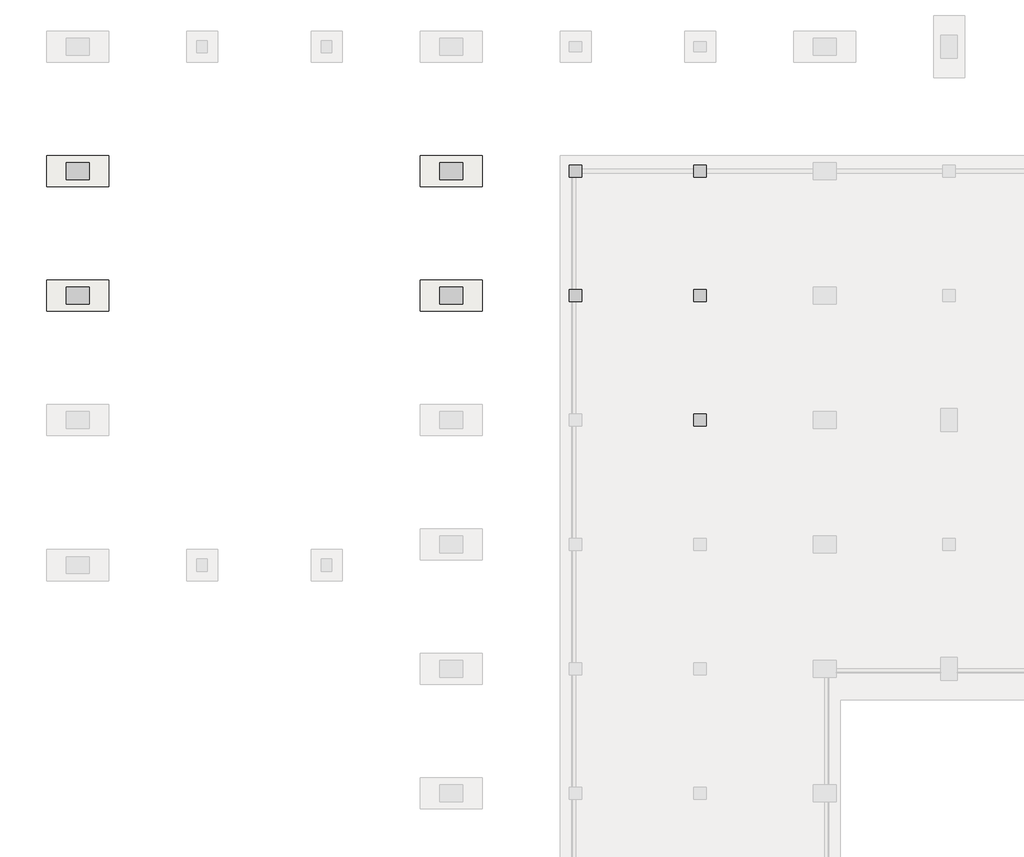
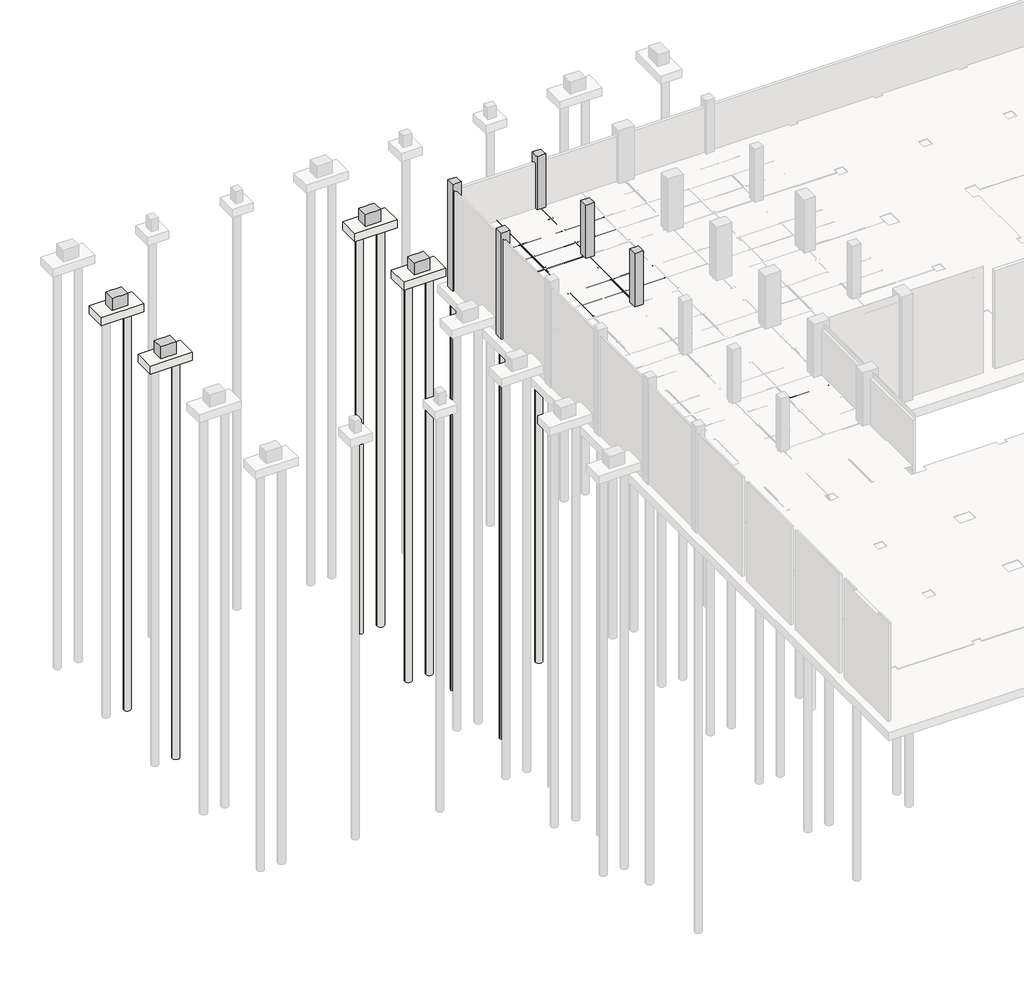
# Not in any storey, part 8 of 16: 24 beams, 13 slabs, 9 columns.
"""IFC4 building model written with IfcOpenShell, lengths in millimetres."""

import ifcopenshell
import ifcopenshell.guid

model = None  # the IFC model being written
_history = None  # IfcOwnerHistory: only IFC2X3 demands one
_inside = {}  # id of a spatial element -> (the spatial element, [elements in it])
_under = {}  # id of a project, library or spatial element -> (it, [spatial elements below it])
_declared = {}  # id of a project -> (the project, [libraries it declares])
_typed = {}  # id of a type object -> (the type object, [elements of that type])
_made_of = {}  # id of a material, layer set ... -> (it, [elements and type objects made of it])


def new_model(schema):
    """Start an empty IFC model of exactly this schema.

    Asked for "IFC4X3", IfcOpenShell would pick the latest addendum, in which some entities
    have other attributes; the version numbers below select the first issue.
    IFC2X3 requires an IfcOwnerHistory on every rooted entity: one is made here for all.
    """
    global model, _history
    if schema == "IFC4X3":
        model = ifcopenshell.file(schema_version=(4, 3, 0, 0))
    else:
        model = ifcopenshell.file(schema=schema)
    _inside.clear()
    _under.clear()
    _declared.clear()
    _typed.clear()
    _made_of.clear()
    _history = None
    if model.schema == "IFC2X3":
        org = make("IfcOrganization", Name="unknown")
        user = make(
            "IfcPersonAndOrganization",
            ThePerson=make("IfcPerson", FamilyName="unknown"),
            TheOrganization=org,
        )
        app = make(
            "IfcApplication",
            ApplicationDeveloper=org,
            Version="unknown",
            ApplicationFullName="unknown",
            ApplicationIdentifier="unknown",
        )
        _history = make(
            "IfcOwnerHistory",
            OwningUser=user,
            OwningApplication=app,
            ChangeAction="ADDED",
            CreationDate=0,
        )
    return model


def make(cls, **values):
    """One entity of the class cls with the attributes given. An attribute that is None is left unset."""
    return model.create_entity(
        cls, **{name: value for name, value in values.items() if value is not None}
    )


def rooted(cls, **values):
    """An entity with a GlobalId (a new one), such as an element, a storey or a relation."""
    return make(cls, GlobalId=ifcopenshell.guid.new(), OwnerHistory=_history, **values)


def si_unit(unit_type, name, prefix=None):
    """IfcSIUnit, for example si_unit("LENGTHUNIT", "METRE", prefix="MILLI")."""
    return make("IfcSIUnit", UnitType=unit_type, Prefix=prefix, Name=name)


def assignment(units):
    """IfcUnitAssignment: the units of a project."""
    return None if units is None else make("IfcUnitAssignment", Units=units)


def point(xyz):
    """IfcCartesianPoint."""
    return None if xyz is None else make("IfcCartesianPoint", Coordinates=xyz)


def direction(xyz):
    """IfcDirection."""
    return None if xyz is None else make("IfcDirection", DirectionRatios=xyz)


def frame(location, z_axis=None, x_axis=None):
    """IfcAxis2Placement3D, a coordinate frame: its origin and axes. An axis left out is left unset."""
    return make(
        "IfcAxis2Placement3D",
        Location=point(location),
        Axis=direction(z_axis),
        RefDirection=direction(x_axis),
    )


def frame_2d(location, x_axis=None):
    """IfcAxis2Placement2D, a coordinate frame in the plane: its origin and x axis."""
    return make(
        "IfcAxis2Placement2D", Location=point(location), RefDirection=direction(x_axis)
    )


def origin():
    """The frame at (0, 0, 0) with its axes left unset."""
    return frame((0.0, 0.0, 0.0))


def place(relative_to, where):
    """IfcLocalPlacement: puts the frame where relative to a parent placement (None: the world)."""
    return make(
        "IfcLocalPlacement", PlacementRelTo=relative_to, RelativePlacement=where
    )


def context(
    kind, dimensions, precision=None, world=None, true_north=None, identifier=None
):
    """IfcGeometricRepresentationContext, for example the 3D "Model" context."""
    return make(
        "IfcGeometricRepresentationContext",
        ContextIdentifier=identifier,
        ContextType=kind,
        CoordinateSpaceDimension=dimensions,
        Precision=precision,
        WorldCoordinateSystem=world,
        TrueNorth=true_north,
    )


def project(units=None, contexts=None):
    """IfcProject with its units and contexts."""
    return rooted(
        "IfcProject",
        Name="project",
        RepresentationContexts=contexts,
        UnitsInContext=assignment(units),
    )


def spatial(cls, under=None, at=None, **own):
    """A site, building, storey or space (cls), placed at a placement, below another one or the project."""
    s = rooted(cls, ObjectPlacement=at, **own)
    if under is not None:
        _under.setdefault(under.id(), (under, []))[1].append(s)
    return s


def polyline(points):
    """IfcPolyline through the points."""
    return make("IfcPolyline", Points=[point(p) for p in points])


def circle_curve(where, radius):
    """IfcCircle in the frame where."""
    return make("IfcCircle", Position=where, Radius=radius)


def trimmed(basis, trim1, trim2, sense, master):
    """IfcTrimmedCurve: the piece of a basis curve between two trims."""
    return make(
        "IfcTrimmedCurve",
        BasisCurve=basis,
        Trim1=trim1,
        Trim2=trim2,
        SenseAgreement=sense,
        MasterRepresentation=master,
    )


def segment(curve, same_sense, transition):
    """IfcCompositeCurveSegment."""
    return make(
        "IfcCompositeCurveSegment",
        Transition=transition,
        SameSense=same_sense,
        ParentCurve=curve,
    )


def composite_curve(segments, self_intersect=None):
    """IfcCompositeCurve: segments joined end to end."""
    return make("IfcCompositeCurve", Segments=segments, SelfIntersect=self_intersect)


def outline(outer, holes=None, kind="AREA"):
    """IfcArbitraryClosedProfileDef: a profile drawn as a closed curve; with holes, ...WithVoids."""
    if holes is None:
        return make("IfcArbitraryClosedProfileDef", ProfileType=kind, OuterCurve=outer)
    return make(
        "IfcArbitraryProfileDefWithVoids",
        ProfileType=kind,
        OuterCurve=outer,
        InnerCurves=holes,
    )


def extrude(swept, where, along, depth):
    """IfcExtrudedAreaSolid: the profile swept, set in the frame where, extruded along a direction by depth."""
    return make(
        "IfcExtrudedAreaSolid",
        SweptArea=swept,
        Position=where,
        ExtrudedDirection=direction(along),
        Depth=depth,
    )


def faces_of(points, faces, orient=None, outer=None):
    """IfcFace entities. A face is a list of loops; a loop is a list of indices into points, from 0.

    orient and outer hold one flag for each loop. By default every Orientation is true, the
    first loop of a face is its IfcFaceOuterBound and the others are IfcFaceBound.
    """
    made = []
    for i, loops in enumerate(faces):
        bounds = []
        for j, loop in enumerate(loops):
            is_outer = j == 0 if outer is None else outer[i][j]
            bounds.append(
                make(
                    "IfcFaceOuterBound" if is_outer else "IfcFaceBound",
                    Bound=make("IfcPolyLoop", Polygon=[points[k] for k in loop]),
                    Orientation=True if orient is None else orient[i][j],
                )
            )
        made.append(make("IfcFace", Bounds=bounds))
    return made


def faceted_brep(points, faces, orient=None, outer=None, voids=None):
    """IfcFacetedBrep: a solid bounded by flat faces; with voids (closed shells), ...WithVoids."""
    shared = [point(p) for p in points]
    hull = make("IfcClosedShell", CfsFaces=faces_of(shared, faces, orient, outer))
    if voids is None:
        return make("IfcFacetedBrep", Outer=hull)
    return make(
        "IfcFacetedBrepWithVoids",
        Outer=hull,
        Voids=[
            make(cls, CfsFaces=faces_of(shared, fs, o, b)) for cls, fs, o, b in voids
        ],
    )


def shape(context_of_items, identifier, shape_type, items):
    """IfcShapeRepresentation: the items that make up one representation, for example the "Body"."""
    return make(
        "IfcShapeRepresentation",
        ContextOfItems=context_of_items,
        RepresentationIdentifier=identifier,
        RepresentationType=shape_type,
        Items=items,
    )


def made_of(thing, what):
    """Note that an element or type object is made of a material, layer set ...; save() writes the relation."""
    if what is not None:
        _made_of.setdefault(what.id(), (what, []))[1].append(thing)
    return thing


def element(
    cls,
    number,
    at=None,
    inside=None,
    cuts=None,
    type_object=None,
    material=None,
    context=None,
    identifier="Body",
    shape_type=None,
    held_by="IfcProductDefinitionShape",
    body=None,
    shapes=None,
    **own,
):
    """One element of the class cls, such as IfcWall. Its Tag is "e" and its number.

    at: its placement. inside: the storey or other place that contains it. cuts: it is an
    opening in that element (IfcRelVoidsElement). A single representation is given by context,
    identifier, shape_type and body (its items); several are given by shapes. held_by: the class
    of the entity that holds the representations. save() writes the other relations.
    """
    e = rooted(cls, Tag="e%d" % number, ObjectPlacement=at, **own)
    if body is not None:
        shapes = [shape(context, identifier, shape_type, body)]
    if shapes is not None:
        e.Representation = make(held_by, Representations=shapes)
    if inside is not None:
        _inside.setdefault(inside.id(), (inside, []))[1].append(e)
    if cuts is not None:
        rooted(
            "IfcRelVoidsElement", RelatingBuildingElement=cuts, RelatedOpeningElement=e
        )
    if type_object is not None:
        _typed.setdefault(type_object.id(), (type_object, []))[1].append(e)
    return made_of(e, material)


def aggregate(whole, parts):
    """IfcRelAggregates: a whole, such as a stair, and the parts it consists of."""
    return rooted("IfcRelAggregates", RelatingObject=whole, RelatedObjects=parts)


def save(model, path):
    """Write the relations noted so far, then the file.

    IfcRelAggregates (storeys below a building ...), IfcRelContainedInSpatialStructure (elements
    in a storey), IfcRelDefinesByType, IfcRelAssociatesMaterial and IfcRelDeclares: one each for
    every whole, place, type object, material and project.
    """
    for whole, parts in _under.values():
        aggregate(whole, parts)
    for where, things in _inside.values():
        rooted(
            "IfcRelContainedInSpatialStructure",
            RelatedElements=things,
            RelatingStructure=where,
        )
    for kind, things in _typed.values():
        rooted("IfcRelDefinesByType", RelatedObjects=things, RelatingType=kind)
    for what, things in _made_of.values():
        rooted("IfcRelAssociatesMaterial", RelatedObjects=things, RelatingMaterial=what)
    for by, libraries in _declared.values():
        rooted("IfcRelDeclares", RelatingContext=by, RelatedDefinitions=libraries)
    model.write(path)


model = new_model("IFC4")

# Units and contexts
model_context = context("Model", 3, world=origin())
ifc_project = project(units=[si_unit("LENGTHUNIT", "METRE", prefix="MILLI")], contexts=[model_context])

# Site, building
site = spatial("IfcSite", under=ifc_project)
building = spatial("IfcBuilding", under=site)

# Beams
placement = place(None, origin())
element("IfcBeam", 1, at=placement, inside=building, context=model_context, shape_type="SweptSolid", body=[
    extrude(outline(composite_curve([segment(polyline([(-11900.0, -4187.0381366), (-11900.0, -4200.0381366), (-12100.0, -4200.0381366), (-12100.0, -4187.0381366), (-12020.0, -4187.0381366)]), True, "CONTINUOUS"), segment(trimmed(circle_curve(frame_2d((-12020.0, -4171.0381366)), 16.0), [point((-12020.0, -4187.0381366))], [point((-12004.0, -4171.0381366))], True, "CARTESIAN"), True, "CONTINUOUS"), segment(polyline([(-12004.0, -4171.0381366), (-12004.0, -3829.0381366)]), True, "CONTINUOUS"), segment(trimmed(circle_curve(frame_2d((-12020.0, -3829.0381366)), 16.0), [point((-12004.0, -3829.0381366))], [point((-12020.0, -3813.0381366))], True, "CARTESIAN"), True, "CONTINUOUS"), segment(polyline([(-12020.0, -3813.0381366), (-12100.0, -3813.0381366), (-12100.0, -3800.0381366), (-11900.0, -3800.0381366), (-11900.0, -3813.0381366), (-11980.0, -3813.0381366)]), True, "CONTINUOUS"), segment(trimmed(circle_curve(frame_2d((-11980.0, -3829.0381366)), 16.0), [point((-11980.0, -3813.0381366))], [point((-11996.0, -3829.0381366))], True, "CARTESIAN"), True, "CONTINUOUS"), segment(polyline([(-11996.0, -3829.0381366), (-11996.0, -4171.0381366)]), True, "CONTINUOUS"), segment(trimmed(circle_curve(frame_2d((-11980.0, -4171.0381366)), 16.0), [point((-11996.0, -4171.0381366))], [point((-11980.0, -4187.0381366))], True, "CARTESIAN"), True, "CONTINUOUS"), segment(polyline([(-11980.0, -4187.0381366), (-11900.0, -4187.0381366)]), True, "CONTINUOUS")], self_intersect=False)), frame((24312.7, 0.0, 0.0), z_axis=(1.0, 0.0, 0.0), x_axis=(0.0, 1.0, 0.0)), (0.0, 0.0, 1.0), 5374.6),
])
element("IfcBeam", 2, at=placement, inside=building, context=model_context, shape_type="SweptSolid", body=[
    extrude(outline(composite_curve([segment(polyline([(-4187.0381366, 29900.0), (-4200.0381366, 29900.0), (-4200.0381366, 30100.0), (-4187.0381366, 30100.0), (-4187.0381366, 30020.0)]), True, "CONTINUOUS"), segment(trimmed(circle_curve(frame_2d((-4171.0381366, 30020.0)), 16.0), [point((-4187.0381366, 30020.0))], [point((-4171.0381366, 30004.0))], True, "CARTESIAN"), True, "CONTINUOUS"), segment(polyline([(-4171.0381366, 30004.0), (-3829.0381366, 30004.0)]), True, "CONTINUOUS"), segment(trimmed(circle_curve(frame_2d((-3829.0381366, 30020.0)), 16.0), [point((-3829.0381366, 30004.0))], [point((-3813.0381366, 30020.0))], True, "CARTESIAN"), True, "CONTINUOUS"), segment(polyline([(-3813.0381366, 30020.0), (-3813.0381366, 30100.0), (-3800.0381366, 30100.0), (-3800.0381366, 29900.0), (-3813.0381366, 29900.0), (-3813.0381366, 29980.0)]), True, "CONTINUOUS"), segment(trimmed(circle_curve(frame_2d((-3829.0381366, 29980.0)), 16.0), [point((-3813.0381366, 29980.0))], [point((-3829.0381366, 29996.0))], True, "CARTESIAN"), True, "CONTINUOUS"), segment(polyline([(-3829.0381366, 29996.0), (-4171.0381366, 29996.0)]), True, "CONTINUOUS"), segment(trimmed(circle_curve(frame_2d((-4171.0381366, 29980.0)), 16.0), [point((-4171.0381366, 29996.0))], [point((-4187.0381366, 29980.0))], True, "CARTESIAN"), True, "CONTINUOUS"), segment(polyline([(-4187.0381366, 29980.0), (-4187.0381366, 29900.0)]), True, "CONTINUOUS")], self_intersect=False)), frame((0.0, -11687.3, 0.0), z_axis=(0.0, 1.0, 0.0), x_axis=(0.0, 0.0, 1.0)), (0.0, 0.0, 1.0), 5374.6),
])
element("IfcBeam", 3, at=placement, inside=building, context=model_context, shape_type="SweptSolid", body=[
    extrude(outline(composite_curve([segment(polyline([(-4187.0381366, 26900.0), (-4200.0381366, 26900.0), (-4200.0381366, 27100.0), (-4187.0381366, 27100.0), (-4187.0381366, 27020.0)]), True, "CONTINUOUS"), segment(trimmed(circle_curve(frame_2d((-4171.0381366, 27020.0)), 16.0), [point((-4187.0381366, 27020.0))], [point((-4171.0381366, 27004.0))], True, "CARTESIAN"), True, "CONTINUOUS"), segment(polyline([(-4171.0381366, 27004.0), (-3829.0381366, 27004.0)]), True, "CONTINUOUS"), segment(trimmed(circle_curve(frame_2d((-3829.0381366, 27020.0)), 16.0), [point((-3829.0381366, 27004.0))], [point((-3813.0381366, 27020.0))], True, "CARTESIAN"), True, "CONTINUOUS"), segment(polyline([(-3813.0381366, 27020.0), (-3813.0381366, 27100.0), (-3800.0381366, 27100.0), (-3800.0381366, 26900.0), (-3813.0381366, 26900.0), (-3813.0381366, 26980.0)]), True, "CONTINUOUS"), segment(trimmed(circle_curve(frame_2d((-3829.0381366, 26980.0)), 16.0), [point((-3813.0381366, 26980.0))], [point((-3829.0381366, 26996.0))], True, "CARTESIAN"), True, "CONTINUOUS"), segment(polyline([(-3829.0381366, 26996.0), (-4171.0381366, 26996.0)]), True, "CONTINUOUS"), segment(trimmed(circle_curve(frame_2d((-4171.0381366, 26980.0)), 16.0), [point((-4171.0381366, 26996.0))], [point((-4187.0381366, 26980.0))], True, "CARTESIAN"), True, "CONTINUOUS"), segment(polyline([(-4187.0381366, 26980.0), (-4187.0381366, 26900.0)]), True, "CONTINUOUS")], self_intersect=False)), frame((0.0, -11887.3, 0.0), z_axis=(0.0, 1.0, 0.0), x_axis=(0.0, 0.0, 1.0)), (0.0, 0.0, 1.0), 5887.3),
])
element("IfcBeam", 4, at=placement, inside=building, context=model_context, shape_type="SweptSolid", body=[
    extrude(outline(composite_curve([segment(polyline([(-8977.2, -3800.0381366), (-8977.2, -3950.0381366), (-9052.2, -3950.0381366)]), True, "CONTINUOUS"), segment(trimmed(circle_curve(frame_2d((-9042.2, -3950.0381366)), 10.0), [point((-9052.2, -3950.0381366))], [point((-9042.2, -3940.0381366))], False, "CARTESIAN"), True, "CONTINUOUS"), segment(polyline([(-9042.2, -3940.0381366), (-8983.7, -3930.7726469), (-8983.7, -3819.3036264), (-9042.2, -3810.0381366)]), True, "CONTINUOUS"), segment(trimmed(circle_curve(frame_2d((-9042.2, -3800.0381366)), 10.0), [point((-9042.2, -3810.0381366))], [point((-9052.2, -3800.0381366))], False, "CARTESIAN"), True, "CONTINUOUS"), segment(polyline([(-9052.2, -3800.0381366), (-8977.2, -3800.0381366)]), True, "CONTINUOUS")], self_intersect=False)), frame((24000.0, 0.0, 0.0), z_axis=(1.0, 0.0, 0.0), x_axis=(0.0, 1.0, 0.0)), (0.0, 0.0, 1.0), 2887.3),
])
element("IfcBeam", 5, at=placement, inside=building, context=model_context, shape_type="SweptSolid", body=[
    extrude(outline(composite_curve([segment(polyline([(-10477.2, -3800.0381366), (-10477.2, -3950.0381366), (-10552.2, -3950.0381366)]), True, "CONTINUOUS"), segment(trimmed(circle_curve(frame_2d((-10542.2, -3950.0381366)), 10.0), [point((-10552.2, -3950.0381366))], [point((-10542.2, -3940.0381366))], False, "CARTESIAN"), True, "CONTINUOUS"), segment(polyline([(-10542.2, -3940.0381366), (-10483.7, -3930.7726469), (-10483.7, -3819.3036264), (-10542.2, -3810.0381366)]), True, "CONTINUOUS"), segment(trimmed(circle_curve(frame_2d((-10542.2, -3800.0381366)), 10.0), [point((-10542.2, -3810.0381366))], [point((-10552.2, -3800.0381366))], False, "CARTESIAN"), True, "CONTINUOUS"), segment(polyline([(-10552.2, -3800.0381366), (-10477.2, -3800.0381366)]), True, "CONTINUOUS")], self_intersect=False)), frame((24000.0, 0.0, 0.0), z_axis=(1.0, 0.0, 0.0), x_axis=(0.0, 1.0, 0.0)), (0.0, 0.0, 1.0), 2887.3),
])
element("IfcBeam", 6, at=placement, inside=building, context=model_context, shape_type="SweptSolid", body=[
    extrude(outline(composite_curve([segment(polyline([(-7477.2, -3800.0381366), (-7477.2, -3950.0381366), (-7552.2, -3950.0381366)]), True, "CONTINUOUS"), segment(trimmed(circle_curve(frame_2d((-7542.2, -3950.0381366)), 10.0), [point((-7552.2, -3950.0381366))], [point((-7542.2, -3940.0381366))], False, "CARTESIAN"), True, "CONTINUOUS"), segment(polyline([(-7542.2, -3940.0381366), (-7483.7, -3930.7726469), (-7483.7, -3819.3036264), (-7542.2, -3810.0381366)]), True, "CONTINUOUS"), segment(trimmed(circle_curve(frame_2d((-7542.2, -3800.0381366)), 10.0), [point((-7542.2, -3810.0381366))], [point((-7552.2, -3800.0381366))], False, "CARTESIAN"), True, "CONTINUOUS"), segment(polyline([(-7552.2, -3800.0381366), (-7477.2, -3800.0381366)]), True, "CONTINUOUS")], self_intersect=False)), frame((24000.0, 0.0, 0.0), z_axis=(1.0, 0.0, 0.0), x_axis=(0.0, 1.0, 0.0)), (0.0, 0.0, 1.0), 2887.3),
])
element("IfcBeam", 7, at=placement, inside=building, context=model_context, shape_type="SweptSolid", body=[
    extrude(outline(composite_curve([segment(polyline([(-8977.2, -3800.0381366), (-8977.2, -3950.0381366), (-9052.2, -3950.0381366)]), True, "CONTINUOUS"), segment(trimmed(circle_curve(frame_2d((-9042.2, -3950.0381366)), 10.0), [point((-9052.2, -3950.0381366))], [point((-9042.2, -3940.0381366))], False, "CARTESIAN"), True, "CONTINUOUS"), segment(polyline([(-9042.2, -3940.0381366), (-8983.7, -3930.7726469), (-8983.7, -3819.3036264), (-9042.2, -3810.0381366)]), True, "CONTINUOUS"), segment(trimmed(circle_curve(frame_2d((-9042.2, -3800.0381366)), 10.0), [point((-9042.2, -3810.0381366))], [point((-9052.2, -3800.0381366))], False, "CARTESIAN"), True, "CONTINUOUS"), segment(polyline([(-9052.2, -3800.0381366), (-8977.2, -3800.0381366)]), True, "CONTINUOUS")], self_intersect=False)), frame((27112.7, 0.0, 0.0), z_axis=(1.0, 0.0, 0.0), x_axis=(0.0, 1.0, 0.0)), (0.0, 0.0, 1.0), 2774.6),
])
element("IfcBeam", 8, at=placement, inside=building, context=model_context, shape_type="SweptSolid", body=[
    extrude(outline(composite_curve([segment(polyline([(-10477.2, -3800.0381366), (-10477.2, -3950.0381366), (-10552.2, -3950.0381366)]), True, "CONTINUOUS"), segment(trimmed(circle_curve(frame_2d((-10542.2, -3950.0381366)), 10.0), [point((-10552.2, -3950.0381366))], [point((-10542.2, -3940.0381366))], False, "CARTESIAN"), True, "CONTINUOUS"), segment(polyline([(-10542.2, -3940.0381366), (-10483.7, -3930.7726469), (-10483.7, -3819.3036264), (-10542.2, -3810.0381366)]), True, "CONTINUOUS"), segment(trimmed(circle_curve(frame_2d((-10542.2, -3800.0381366)), 10.0), [point((-10542.2, -3810.0381366))], [point((-10552.2, -3800.0381366))], False, "CARTESIAN"), True, "CONTINUOUS"), segment(polyline([(-10552.2, -3800.0381366), (-10477.2, -3800.0381366)]), True, "CONTINUOUS")], self_intersect=False)), frame((27112.7, 0.0, 0.0), z_axis=(1.0, 0.0, 0.0), x_axis=(0.0, 1.0, 0.0)), (0.0, 0.0, 1.0), 2774.6),
])
element("IfcBeam", 9, at=placement, inside=building, context=model_context, shape_type="SweptSolid", body=[
    extrude(outline(composite_curve([segment(polyline([(-7477.2, -3800.0381366), (-7477.2, -3950.0381366), (-7552.2, -3950.0381366)]), True, "CONTINUOUS"), segment(trimmed(circle_curve(frame_2d((-7542.2, -3950.0381366)), 10.0), [point((-7552.2, -3950.0381366))], [point((-7542.2, -3940.0381366))], False, "CARTESIAN"), True, "CONTINUOUS"), segment(polyline([(-7542.2, -3940.0381366), (-7483.7, -3930.7726469), (-7483.7, -3819.3036264), (-7542.2, -3810.0381366)]), True, "CONTINUOUS"), segment(trimmed(circle_curve(frame_2d((-7542.2, -3800.0381366)), 10.0), [point((-7542.2, -3810.0381366))], [point((-7552.2, -3800.0381366))], False, "CARTESIAN"), True, "CONTINUOUS"), segment(polyline([(-7552.2, -3800.0381366), (-7477.2, -3800.0381366)]), True, "CONTINUOUS")], self_intersect=False)), frame((27112.7, 0.0, 0.0), z_axis=(1.0, 0.0, 0.0), x_axis=(0.0, 1.0, 0.0)), (0.0, 0.0, 1.0), 2774.6),
])
element("IfcBeam", 10, at=placement, inside=building, context=model_context, shape_type="SweptSolid", body=[
    extrude(outline(composite_curve([segment(polyline([(-8977.2, -3800.0381366), (-8977.2, -3950.0381366), (-9052.2, -3950.0381366)]), True, "CONTINUOUS"), segment(trimmed(circle_curve(frame_2d((-9042.2, -3950.0381366)), 10.0), [point((-9052.2, -3950.0381366))], [point((-9042.2, -3940.0381366))], False, "CARTESIAN"), True, "CONTINUOUS"), segment(polyline([(-9042.2, -3940.0381366), (-8983.7, -3930.7726469), (-8983.7, -3819.3036264), (-9042.2, -3810.0381366)]), True, "CONTINUOUS"), segment(trimmed(circle_curve(frame_2d((-9042.2, -3800.0381366)), 10.0), [point((-9042.2, -3810.0381366))], [point((-9052.2, -3800.0381366))], False, "CARTESIAN"), True, "CONTINUOUS"), segment(polyline([(-9052.2, -3800.0381366), (-8977.2, -3800.0381366)]), True, "CONTINUOUS")], self_intersect=False)), frame((30112.7, 0.0, 0.0), z_axis=(1.0, 0.0, 0.0), x_axis=(0.0, 1.0, 0.0)), (0.0, 0.0, 1.0), 2774.6),
])
element("IfcBeam", 11, at=placement, inside=building, context=model_context, shape_type="SweptSolid", body=[
    extrude(outline(composite_curve([segment(polyline([(-10477.2, -3800.0381366), (-10477.2, -3950.0381366), (-10552.2, -3950.0381366)]), True, "CONTINUOUS"), segment(trimmed(circle_curve(frame_2d((-10542.2, -3950.0381366)), 10.0), [point((-10552.2, -3950.0381366))], [point((-10542.2, -3940.0381366))], False, "CARTESIAN"), True, "CONTINUOUS"), segment(polyline([(-10542.2, -3940.0381366), (-10483.7, -3930.7726469), (-10483.7, -3819.3036264), (-10542.2, -3810.0381366)]), True, "CONTINUOUS"), segment(trimmed(circle_curve(frame_2d((-10542.2, -3800.0381366)), 10.0), [point((-10542.2, -3810.0381366))], [point((-10552.2, -3800.0381366))], False, "CARTESIAN"), True, "CONTINUOUS"), segment(polyline([(-10552.2, -3800.0381366), (-10477.2, -3800.0381366)]), True, "CONTINUOUS")], self_intersect=False)), frame((30112.7, 0.0, 0.0), z_axis=(1.0, 0.0, 0.0), x_axis=(0.0, 1.0, 0.0)), (0.0, 0.0, 1.0), 2774.6),
])
element("IfcBeam", 12, at=placement, inside=building, context=model_context, shape_type="SweptSolid", body=[
    extrude(outline(composite_curve([segment(polyline([(-7477.2, -3800.0381366), (-7477.2, -3950.0381366), (-7552.2, -3950.0381366)]), True, "CONTINUOUS"), segment(trimmed(circle_curve(frame_2d((-7542.2, -3950.0381366)), 10.0), [point((-7552.2, -3950.0381366))], [point((-7542.2, -3940.0381366))], False, "CARTESIAN"), True, "CONTINUOUS"), segment(polyline([(-7542.2, -3940.0381366), (-7483.7, -3930.7726469), (-7483.7, -3819.3036264), (-7542.2, -3810.0381366)]), True, "CONTINUOUS"), segment(trimmed(circle_curve(frame_2d((-7542.2, -3800.0381366)), 10.0), [point((-7542.2, -3810.0381366))], [point((-7552.2, -3800.0381366))], False, "CARTESIAN"), True, "CONTINUOUS"), segment(polyline([(-7552.2, -3800.0381366), (-7477.2, -3800.0381366)]), True, "CONTINUOUS")], self_intersect=False)), frame((30112.7, 0.0, 0.0), z_axis=(1.0, 0.0, 0.0), x_axis=(0.0, 1.0, 0.0)), (0.0, 0.0, 1.0), 2774.6),
])
element("IfcBeam", 13, at=placement, inside=building, context=model_context, shape_type="SweptSolid", body=[
    extrude(outline(composite_curve([segment(polyline([(-4187.0381366, 29900.0), (-4200.0381366, 29900.0), (-4200.0381366, 30100.0), (-4187.0381366, 30100.0), (-4187.0381366, 30020.0)]), True, "CONTINUOUS"), segment(trimmed(circle_curve(frame_2d((-4171.0381366, 30020.0)), 16.0), [point((-4187.0381366, 30020.0))], [point((-4171.0381366, 30004.0))], True, "CARTESIAN"), True, "CONTINUOUS"), segment(polyline([(-4171.0381366, 30004.0), (-3829.0381366, 30004.0)]), True, "CONTINUOUS"), segment(trimmed(circle_curve(frame_2d((-3829.0381366, 30020.0)), 16.0), [point((-3829.0381366, 30004.0))], [point((-3813.0381366, 30020.0))], True, "CARTESIAN"), True, "CONTINUOUS"), segment(polyline([(-3813.0381366, 30020.0), (-3813.0381366, 30100.0), (-3800.0381366, 30100.0), (-3800.0381366, 29900.0), (-3813.0381366, 29900.0), (-3813.0381366, 29980.0)]), True, "CONTINUOUS"), segment(trimmed(circle_curve(frame_2d((-3829.0381366, 29980.0)), 16.0), [point((-3813.0381366, 29980.0))], [point((-3829.0381366, 29996.0))], True, "CARTESIAN"), True, "CONTINUOUS"), segment(polyline([(-3829.0381366, 29996.0), (-4171.0381366, 29996.0)]), True, "CONTINUOUS"), segment(trimmed(circle_curve(frame_2d((-4171.0381366, 29980.0)), 16.0), [point((-4171.0381366, 29996.0))], [point((-4187.0381366, 29980.0))], True, "CARTESIAN"), True, "CONTINUOUS"), segment(polyline([(-4187.0381366, 29980.0), (-4187.0381366, 29900.0)]), True, "CONTINUOUS")], self_intersect=False)), frame((0.0, -17687.3, 0.0), z_axis=(0.0, 1.0, 0.0), x_axis=(0.0, 0.0, 1.0)), (0.0, 0.0, 1.0), 5374.6),
])
element("IfcBeam", 14, at=placement, inside=building, context=model_context, shape_type="SweptSolid", body=[
    extrude(outline(composite_curve([segment(polyline([(-4187.0381366, 26900.0), (-4200.0381366, 26900.0), (-4200.0381366, 27100.0), (-4187.0381366, 27100.0), (-4187.0381366, 27020.0)]), True, "CONTINUOUS"), segment(trimmed(circle_curve(frame_2d((-4171.0381366, 27020.0)), 16.0), [point((-4187.0381366, 27020.0))], [point((-4171.0381366, 27004.0))], True, "CARTESIAN"), True, "CONTINUOUS"), segment(polyline([(-4171.0381366, 27004.0), (-3829.0381366, 27004.0)]), True, "CONTINUOUS"), segment(trimmed(circle_curve(frame_2d((-3829.0381366, 27020.0)), 16.0), [point((-3829.0381366, 27004.0))], [point((-3813.0381366, 27020.0))], True, "CARTESIAN"), True, "CONTINUOUS"), segment(polyline([(-3813.0381366, 27020.0), (-3813.0381366, 27100.0), (-3800.0381366, 27100.0), (-3800.0381366, 26900.0), (-3813.0381366, 26900.0), (-3813.0381366, 26980.0)]), True, "CONTINUOUS"), segment(trimmed(circle_curve(frame_2d((-3829.0381366, 26980.0)), 16.0), [point((-3813.0381366, 26980.0))], [point((-3829.0381366, 26996.0))], True, "CARTESIAN"), True, "CONTINUOUS"), segment(polyline([(-3829.0381366, 26996.0), (-4171.0381366, 26996.0)]), True, "CONTINUOUS"), segment(trimmed(circle_curve(frame_2d((-4171.0381366, 26980.0)), 16.0), [point((-4171.0381366, 26996.0))], [point((-4187.0381366, 26980.0))], True, "CARTESIAN"), True, "CONTINUOUS"), segment(polyline([(-4187.0381366, 26980.0), (-4187.0381366, 26900.0)]), True, "CONTINUOUS")], self_intersect=False)), frame((0.0, -17887.3, 0.0), z_axis=(0.0, 1.0, 0.0), x_axis=(0.0, 0.0, 1.0)), (0.0, 0.0, 1.0), 5774.6),
])
element("IfcBeam", 15, at=placement, inside=building, context=model_context, shape_type="SweptSolid", body=[
    extrude(outline(composite_curve([segment(polyline([(-14977.2, -3800.0381366), (-14977.2, -3950.0381366), (-15052.2, -3950.0381366)]), True, "CONTINUOUS"), segment(trimmed(circle_curve(frame_2d((-15042.2, -3950.0381366)), 10.0), [point((-15052.2, -3950.0381366))], [point((-15042.2, -3940.0381366))], False, "CARTESIAN"), True, "CONTINUOUS"), segment(polyline([(-15042.2, -3940.0381366), (-14983.7, -3930.7726469), (-14983.7, -3819.3036264), (-15042.2, -3810.0381366)]), True, "CONTINUOUS"), segment(trimmed(circle_curve(frame_2d((-15042.2, -3800.0381366)), 10.0), [point((-15042.2, -3810.0381366))], [point((-15052.2, -3800.0381366))], False, "CARTESIAN"), True, "CONTINUOUS"), segment(polyline([(-15052.2, -3800.0381366), (-14977.2, -3800.0381366)]), True, "CONTINUOUS")], self_intersect=False)), frame((24000.0, 0.0, 0.0), z_axis=(1.0, 0.0, 0.0), x_axis=(0.0, 1.0, 0.0)), (0.0, 0.0, 1.0), 2887.3),
])
element("IfcBeam", 16, at=placement, inside=building, context=model_context, shape_type="SweptSolid", body=[
    extrude(outline(composite_curve([segment(polyline([(-13477.2, -3800.0381366), (-13477.2, -3950.0381366), (-13552.2, -3950.0381366)]), True, "CONTINUOUS"), segment(trimmed(circle_curve(frame_2d((-13542.2, -3950.0381366)), 10.0), [point((-13552.2, -3950.0381366))], [point((-13542.2, -3940.0381366))], False, "CARTESIAN"), True, "CONTINUOUS"), segment(polyline([(-13542.2, -3940.0381366), (-13483.7, -3930.7726469), (-13483.7, -3819.3036264), (-13542.2, -3810.0381366)]), True, "CONTINUOUS"), segment(trimmed(circle_curve(frame_2d((-13542.2, -3800.0381366)), 10.0), [point((-13542.2, -3810.0381366))], [point((-13552.2, -3800.0381366))], False, "CARTESIAN"), True, "CONTINUOUS"), segment(polyline([(-13552.2, -3800.0381366), (-13477.2, -3800.0381366)]), True, "CONTINUOUS")], self_intersect=False)), frame((24000.0, 0.0, 0.0), z_axis=(1.0, 0.0, 0.0), x_axis=(0.0, 1.0, 0.0)), (0.0, 0.0, 1.0), 2887.3),
])
element("IfcBeam", 17, at=placement, inside=building, context=model_context, shape_type="SweptSolid", body=[
    extrude(outline(composite_curve([segment(polyline([(-14977.2, -3800.0381366), (-14977.2, -3950.0381366), (-15052.2, -3950.0381366)]), True, "CONTINUOUS"), segment(trimmed(circle_curve(frame_2d((-15042.2, -3950.0381366)), 10.0), [point((-15052.2, -3950.0381366))], [point((-15042.2, -3940.0381366))], False, "CARTESIAN"), True, "CONTINUOUS"), segment(polyline([(-15042.2, -3940.0381366), (-14983.7, -3930.7726469), (-14983.7, -3819.3036264), (-15042.2, -3810.0381366)]), True, "CONTINUOUS"), segment(trimmed(circle_curve(frame_2d((-15042.2, -3800.0381366)), 10.0), [point((-15042.2, -3810.0381366))], [point((-15052.2, -3800.0381366))], False, "CARTESIAN"), True, "CONTINUOUS"), segment(polyline([(-15052.2, -3800.0381366), (-14977.2, -3800.0381366)]), True, "CONTINUOUS")], self_intersect=False)), frame((27112.7, 0.0, 0.0), z_axis=(1.0, 0.0, 0.0), x_axis=(0.0, 1.0, 0.0)), (0.0, 0.0, 1.0), 2774.6),
])
element("IfcBeam", 18, at=placement, inside=building, context=model_context, shape_type="SweptSolid", body=[
    extrude(outline(composite_curve([segment(polyline([(-16477.2, -3800.0381366), (-16477.2, -3950.0381366), (-16552.2, -3950.0381366)]), True, "CONTINUOUS"), segment(trimmed(circle_curve(frame_2d((-16542.2, -3950.0381366)), 10.0), [point((-16552.2, -3950.0381366))], [point((-16542.2, -3940.0381366))], False, "CARTESIAN"), True, "CONTINUOUS"), segment(polyline([(-16542.2, -3940.0381366), (-16483.7, -3930.7726469), (-16483.7, -3819.3036264), (-16542.2, -3810.0381366)]), True, "CONTINUOUS"), segment(trimmed(circle_curve(frame_2d((-16542.2, -3800.0381366)), 10.0), [point((-16542.2, -3810.0381366))], [point((-16552.2, -3800.0381366))], False, "CARTESIAN"), True, "CONTINUOUS"), segment(polyline([(-16552.2, -3800.0381366), (-16477.2, -3800.0381366)]), True, "CONTINUOUS")], self_intersect=False)), frame((27112.7, 0.0, 0.0), z_axis=(1.0, 0.0, 0.0), x_axis=(0.0, 1.0, 0.0)), (0.0, 0.0, 1.0), 2774.6),
])
element("IfcBeam", 19, at=placement, inside=building, context=model_context, shape_type="SweptSolid", body=[
    extrude(outline(composite_curve([segment(polyline([(-13477.2, -3800.0381366), (-13477.2, -3950.0381366), (-13552.2, -3950.0381366)]), True, "CONTINUOUS"), segment(trimmed(circle_curve(frame_2d((-13542.2, -3950.0381366)), 10.0), [point((-13552.2, -3950.0381366))], [point((-13542.2, -3940.0381366))], False, "CARTESIAN"), True, "CONTINUOUS"), segment(polyline([(-13542.2, -3940.0381366), (-13483.7, -3930.7726469), (-13483.7, -3819.3036264), (-13542.2, -3810.0381366)]), True, "CONTINUOUS"), segment(trimmed(circle_curve(frame_2d((-13542.2, -3800.0381366)), 10.0), [point((-13542.2, -3810.0381366))], [point((-13552.2, -3800.0381366))], False, "CARTESIAN"), True, "CONTINUOUS"), segment(polyline([(-13552.2, -3800.0381366), (-13477.2, -3800.0381366)]), True, "CONTINUOUS")], self_intersect=False)), frame((27112.7, 0.0, 0.0), z_axis=(1.0, 0.0, 0.0), x_axis=(0.0, 1.0, 0.0)), (0.0, 0.0, 1.0), 2774.6),
])
element("IfcBeam", 20, at=placement, inside=building, context=model_context, shape_type="SweptSolid", body=[
    extrude(outline(composite_curve([segment(polyline([(-14977.2, -3800.0381366), (-14977.2, -3950.0381366), (-15052.2, -3950.0381366)]), True, "CONTINUOUS"), segment(trimmed(circle_curve(frame_2d((-15042.2, -3950.0381366)), 10.0), [point((-15052.2, -3950.0381366))], [point((-15042.2, -3940.0381366))], False, "CARTESIAN"), True, "CONTINUOUS"), segment(polyline([(-15042.2, -3940.0381366), (-14983.7, -3930.7726469), (-14983.7, -3819.3036264), (-15042.2, -3810.0381366)]), True, "CONTINUOUS"), segment(trimmed(circle_curve(frame_2d((-15042.2, -3800.0381366)), 10.0), [point((-15042.2, -3810.0381366))], [point((-15052.2, -3800.0381366))], False, "CARTESIAN"), True, "CONTINUOUS"), segment(polyline([(-15052.2, -3800.0381366), (-14977.2, -3800.0381366)]), True, "CONTINUOUS")], self_intersect=False)), frame((30112.7, 0.0, 0.0), z_axis=(1.0, 0.0, 0.0), x_axis=(0.0, 1.0, 0.0)), (0.0, 0.0, 1.0), 2774.6),
])
element("IfcBeam", 21, at=placement, inside=building, context=model_context, shape_type="SweptSolid", body=[
    extrude(outline(composite_curve([segment(polyline([(-16477.2, -3800.0381366), (-16477.2, -3950.0381366), (-16552.2, -3950.0381366)]), True, "CONTINUOUS"), segment(trimmed(circle_curve(frame_2d((-16542.2, -3950.0381366)), 10.0), [point((-16552.2, -3950.0381366))], [point((-16542.2, -3940.0381366))], False, "CARTESIAN"), True, "CONTINUOUS"), segment(polyline([(-16542.2, -3940.0381366), (-16483.7, -3930.7726469), (-16483.7, -3819.3036264), (-16542.2, -3810.0381366)]), True, "CONTINUOUS"), segment(trimmed(circle_curve(frame_2d((-16542.2, -3800.0381366)), 10.0), [point((-16542.2, -3810.0381366))], [point((-16552.2, -3800.0381366))], False, "CARTESIAN"), True, "CONTINUOUS"), segment(polyline([(-16552.2, -3800.0381366), (-16477.2, -3800.0381366)]), True, "CONTINUOUS")], self_intersect=False)), frame((30112.7, 0.0, 0.0), z_axis=(1.0, 0.0, 0.0), x_axis=(0.0, 1.0, 0.0)), (0.0, 0.0, 1.0), 2774.6),
])
element("IfcBeam", 22, at=placement, inside=building, context=model_context, shape_type="SweptSolid", body=[
    extrude(outline(composite_curve([segment(polyline([(-13477.2, -3800.0381366), (-13477.2, -3950.0381366), (-13552.2, -3950.0381366)]), True, "CONTINUOUS"), segment(trimmed(circle_curve(frame_2d((-13542.2, -3950.0381366)), 10.0), [point((-13552.2, -3950.0381366))], [point((-13542.2, -3940.0381366))], False, "CARTESIAN"), True, "CONTINUOUS"), segment(polyline([(-13542.2, -3940.0381366), (-13483.7, -3930.7726469), (-13483.7, -3819.3036264), (-13542.2, -3810.0381366)]), True, "CONTINUOUS"), segment(trimmed(circle_curve(frame_2d((-13542.2, -3800.0381366)), 10.0), [point((-13542.2, -3810.0381366))], [point((-13552.2, -3800.0381366))], False, "CARTESIAN"), True, "CONTINUOUS"), segment(polyline([(-13552.2, -3800.0381366), (-13477.2, -3800.0381366)]), True, "CONTINUOUS")], self_intersect=False)), frame((30112.7, 0.0, 0.0), z_axis=(1.0, 0.0, 0.0), x_axis=(0.0, 1.0, 0.0)), (0.0, 0.0, 1.0), 2774.6),
])
element("IfcBeam", 23, at=placement, inside=building, context=model_context, shape_type="SweptSolid", body=[
    extrude(outline(composite_curve([segment(polyline([(-19477.2, -3800.0381366), (-19477.2, -3950.0381366), (-19552.2, -3950.0381366)]), True, "CONTINUOUS"), segment(trimmed(circle_curve(frame_2d((-19542.2, -3950.0381366)), 10.0), [point((-19552.2, -3950.0381366))], [point((-19542.2, -3940.0381366))], False, "CARTESIAN"), True, "CONTINUOUS"), segment(polyline([(-19542.2, -3940.0381366), (-19483.7, -3930.7726469), (-19483.7, -3819.3036264), (-19542.2, -3810.0381366)]), True, "CONTINUOUS"), segment(trimmed(circle_curve(frame_2d((-19542.2, -3800.0381366)), 10.0), [point((-19542.2, -3810.0381366))], [point((-19552.2, -3800.0381366))], False, "CARTESIAN"), True, "CONTINUOUS"), segment(polyline([(-19552.2, -3800.0381366), (-19477.2, -3800.0381366)]), True, "CONTINUOUS")], self_intersect=False)), frame((30112.7, 0.0, 0.0), z_axis=(1.0, 0.0, 0.0), x_axis=(0.0, 1.0, 0.0)), (0.0, 0.0, 1.0), 2774.6),
])
element("IfcBeam", 24, at=placement, inside=building, context=model_context, shape_type="SweptSolid", body=[
    extrude(outline(composite_curve([segment(polyline([(-31477.2, -3800.0381366), (-31477.2, -3950.0381366), (-31552.2, -3950.0381366)]), True, "CONTINUOUS"), segment(trimmed(circle_curve(frame_2d((-31542.2, -3950.0381366)), 10.0), [point((-31552.2, -3950.0381366))], [point((-31542.2, -3940.0381366))], False, "CARTESIAN"), True, "CONTINUOUS"), segment(polyline([(-31542.2, -3940.0381366), (-31483.7, -3930.7726469), (-31483.7, -3819.3036264), (-31542.2, -3810.0381366)]), True, "CONTINUOUS"), segment(trimmed(circle_curve(frame_2d((-31542.2, -3800.0381366)), 10.0), [point((-31542.2, -3810.0381366))], [point((-31552.2, -3800.0381366))], False, "CARTESIAN"), True, "CONTINUOUS"), segment(polyline([(-31552.2, -3800.0381366), (-31477.2, -3800.0381366)]), True, "CONTINUOUS")], self_intersect=False)), frame((33112.7, 0.0, 0.0), z_axis=(1.0, 0.0, 0.0), x_axis=(0.0, 1.0, 0.0)), (0.0, 0.0, 1.0), 2774.6),
])

# Columns
element("IfcColumn", 25, ObjectType="RC_Column_Rectangular", at=placement, inside=building, context=model_context, shape_type="Brep", body=[
    faceted_brep([(17450.0, -5600.0, -700.0381366), (18550.0, -5600.0, -700.0381366), (18550.0, -6400.0, -700.0381366), (17450.0, -6400.0, -700.0381366), (17450.0, -5600.0, 199.9618634), (17800.0, -5600.0, 199.9618634), (18200.0, -5600.0, 199.9618634), (18550.0, -5600.0, 199.9618634), (18550.0, -5600.0, -0.0381366), (17450.0, -5600.0, -0.0381366), (18550.0, -6400.0, 199.9618634), (18550.0, -6400.0, -0.0381366), (18200.0, -6400.0, 199.9618634), (17800.0, -6400.0, 199.9618634), (17450.0, -6400.0, 199.9618634), (17450.0, -6400.0, -0.0381366)], [[[0, 1, 2, 3]], [[4, 5, 6, 7, 8, 1, 0, 9]], [[7, 10, 11, 2, 1, 8]], [[10, 12, 13, 14, 15, 3, 2, 11]], [[14, 4, 9, 0, 3, 15]], [[4, 14, 13, 12, 10, 7, 6, 5]]]),
])
element("IfcColumn", 26, ObjectType="RC_Column_Rectangular", at=placement, inside=building, context=model_context, shape_type="Brep", body=[
    faceted_brep([(-550.0, -5600.0, -700.0381366), (550.0, -5600.0, -700.0381366), (550.0, -6400.0, -700.0381366), (-550.0, -6400.0, -700.0381366), (-550.0, -5600.0, 199.9618634), (-200.0, -5600.0, 199.9618634), (200.0, -5600.0, 199.9618634), (550.0, -5600.0, 199.9618634), (550.0, -5600.0, -0.0381366), (550.0, -6400.0, 199.9618634), (550.0, -6400.0, -0.0381366), (200.0, -6400.0, 199.9618634), (-200.0, -6400.0, 199.9618634), (-550.0, -6400.0, 199.9618634)], [[[0, 1, 2, 3]], [[4, 5, 6, 7, 8, 1, 0]], [[7, 9, 10, 2, 1, 8]], [[9, 11, 12, 13, 3, 2, 10]], [[13, 4, 0, 3]], [[4, 13, 12, 11, 9, 7, 6, 5]]]),
])
element("IfcColumn", 27, ObjectType="RC_Column_Rectangular", at=placement, inside=building, context=model_context, shape_type="Brep", body=[
    faceted_brep([(17450.0, -11600.0, -700.0381366), (18550.0, -11600.0, -700.0381366), (18550.0, -12400.0, -700.0381366), (17450.0, -12400.0, -700.0381366), (17450.0, -11600.0, 199.9618634), (17800.0, -11600.0, 199.9618634), (18200.0, -11600.0, 199.9618634), (18550.0, -11600.0, 199.9618634), (18550.0, -11600.0, -0.0381366), (17450.0, -11600.0, -0.0381366), (18550.0, -12400.0, 199.9618634), (18550.0, -12400.0, -0.0381366), (18200.0, -12400.0, 199.9618634), (17800.0, -12400.0, 199.9618634), (17450.0, -12400.0, 199.9618634), (17450.0, -12400.0, -0.0381366)], [[[0, 1, 2, 3]], [[4, 5, 6, 7, 8, 1, 0, 9]], [[7, 10, 11, 2, 1, 8]], [[10, 12, 13, 14, 15, 3, 2, 11]], [[14, 4, 9, 0, 3, 15]], [[4, 14, 13, 12, 10, 7, 6, 5]]]),
])
element("IfcColumn", 28, ObjectType="RC_Column_Rectangular", at=placement, inside=building, context=model_context, shape_type="Brep", body=[
    faceted_brep([(-550.0, -11600.0, -700.0381366), (550.0, -11600.0, -700.0381366), (550.0, -12400.0, -700.0381366), (-550.0, -12400.0, -700.0381366), (-550.0, -11600.0, 199.9618634), (-200.0, -11600.0, 199.9618634), (200.0, -11600.0, 199.9618634), (550.0, -11600.0, 199.9618634), (550.0, -11600.0, -0.0381366), (550.0, -12400.0, 199.9618634), (550.0, -12400.0, -0.0381366), (200.0, -12400.0, 199.9618634), (-200.0, -12400.0, 199.9618634), (-550.0, -12400.0, 199.9618634)], [[[0, 1, 2, 3]], [[4, 5, 6, 7, 8, 1, 0]], [[7, 9, 10, 2, 1, 8]], [[9, 11, 12, 13, 3, 2, 10]], [[13, 4, 0, 3]], [[4, 13, 12, 11, 9, 7, 6, 5]]]),
])
element("IfcColumn", 29, ObjectType="RC_Column_Rectangular", at=placement, inside=building, context=model_context, shape_type="Brep", body=[
    faceted_brep([(30300.0, -5700.0, -7800.0381366), (30300.0, -6300.0, -7800.0381366), (29700.0, -6300.0, -7800.0381366), (29700.0, -5700.0, -7800.0381366), (30300.0, -5700.0, 199.9618634), (30300.0, -6100.0, 199.9618634), (30300.0, -6300.0, 199.9618634), (30300.0, -6300.0, -0.0381366), (30300.0, -6300.0, -3800.0381366), (30300.0, -6300.0, -3832.0381366), (30300.0, -5700.0, -0.0381366), (30175.0, -6300.0, 199.9618634), (29825.0, -6300.0, 199.9618634), (29700.0, -6300.0, 199.9618634), (29700.0, -6300.0, -0.0381366), (29700.0, -6300.0, -3800.0381366), (29700.0, -6300.0, -3832.0381366), (29700.0, -6100.0, 199.9618634), (29700.0, -5700.0, 199.9618634), (29700.0, -5700.0, -0.0381366)], [[[0, 1, 2, 3]], [[4, 5, 6, 7, 8, 9, 1, 0, 10]], [[6, 11, 12, 13, 14, 15, 16, 2, 1, 9, 8, 7]], [[13, 17, 18, 19, 3, 2, 16, 15, 14]], [[18, 4, 10, 0, 3, 19]], [[4, 18, 17, 13, 12, 11, 6, 5]]]),
])
element("IfcColumn", 30, ObjectType="RC_Column_Rectangular", at=placement, inside=building, context=model_context, shape_type="Brep", body=[
    faceted_brep([(24300.0, -5700.0, -7800.0381366), (24300.0, -6300.0, -7800.0381366), (24000.0, -6300.0, -7800.0381366), (23800.0, -6300.0, -7800.0381366), (23700.0, -6300.0, -7800.0381366), (23700.0, -5700.0, -7800.0381366), (24300.0, -5700.0, 199.9618634), (24300.0, -6100.0, 199.9618634), (24300.0, -6300.0, 199.9618634), (24300.0, -6300.0, -0.0381366), (24300.0, -6300.0, -3800.0381366), (24300.0, -6300.0, -3832.0381366), (24300.0, -5700.0, -0.0381366), (24000.0, -6300.0, 199.9618634), (23700.0, -6300.0, 199.9618634), (23700.0, -6300.0, -0.0381366), (23700.0, -5700.0, 199.9618634), (23700.0, -5700.0, -0.0381366)], [[[0, 1, 2, 3, 4, 5]], [[6, 7, 8, 9, 10, 11, 1, 0, 12]], [[8, 13, 14, 15, 4, 3, 2, 1, 11, 10, 9]], [[14, 16, 17, 5, 4, 15]], [[16, 6, 12, 0, 5, 17]], [[6, 16, 14, 13, 8, 7]]]),
])
element("IfcColumn", 31, ObjectType="RC_Column_Rectangular", at=placement, inside=building, context=model_context, shape_type="Brep", body=[
    faceted_brep([(30300.0, -11700.0, -7200.0381366), (30300.0, -12300.0, -7200.0381366), (29700.0, -12300.0, -7200.0381366), (29700.0, -11700.0, -7200.0381366), (30300.0, -11700.0, 199.9618634), (30300.0, -11825.0, 199.9618634), (30300.0, -12175.0, 199.9618634), (30300.0, -12300.0, 199.9618634), (30300.0, -12300.0, -3800.0381366), (30300.0, -12300.0, -3832.0381366), (30300.0, -11700.0, -3832.0381366), (30300.0, -11700.0, -3800.0381366), (30300.0, -11700.0, -0.0381366), (30175.0, -12300.0, 199.9618634), (29825.0, -12300.0, 199.9618634), (29700.0, -12300.0, 199.9618634), (29700.0, -12300.0, -0.0381366), (29700.0, -12300.0, -3800.0381366), (29700.0, -12300.0, -3832.0381366), (29700.0, -12175.0, 199.9618634), (29700.0, -11825.0, 199.9618634), (29700.0, -11700.0, 199.9618634), (29700.0, -11700.0, -0.0381366), (29700.0, -11700.0, -3800.0381366), (29700.0, -11700.0, -3832.0381366), (29825.0, -11700.0, 199.9618634), (30175.0, -11700.0, 199.9618634)], [[[0, 1, 2, 3]], [[4, 5, 6, 7, 8, 9, 1, 0, 10, 11, 12]], [[7, 13, 14, 15, 16, 17, 18, 2, 1, 9, 8]], [[15, 19, 20, 21, 22, 23, 24, 3, 2, 18, 17, 16]], [[21, 25, 26, 4, 12, 11, 10, 0, 3, 24, 23, 22]], [[4, 26, 25, 21, 20, 19, 15, 14, 13, 7, 6, 5]]]),
])
element("IfcColumn", 32, ObjectType="RC_Column_Rectangular", at=placement, inside=building, context=model_context, shape_type="Brep", body=[
    faceted_brep([(24300.0, -11700.0, -7800.0381366), (24300.0, -12300.0, -7800.0381366), (24000.0, -12300.0, -7800.0381366), (23800.0, -12300.0, -7800.0381366), (23700.0, -12300.0, -7800.0381366), (23700.0, -11700.0, -7800.0381366), (23800.0, -11700.0, -7800.0381366), (24000.0, -11700.0, -7800.0381366), (24300.0, -11700.0, 199.9618634), (24300.0, -11825.0, 199.9618634), (24300.0, -12175.0, 199.9618634), (24300.0, -12300.0, 199.9618634), (24300.0, -12300.0, -0.0381366), (24300.0, -12300.0, -3800.0381366), (24300.0, -12300.0, -3832.0381366), (24300.0, -11700.0, -3832.0381366), (24300.0, -11700.0, -3800.0381366), (24300.0, -11700.0, -0.0381366), (24000.0, -12300.0, 199.9618634), (23700.0, -12300.0, 199.9618634), (23700.0, -12300.0, -0.0381366), (23700.0, -11700.0, 199.9618634), (23700.0, -11700.0, -0.0381366), (24000.0, -11700.0, 199.9618634)], [[[0, 1, 2, 3, 4, 5, 6, 7]], [[8, 9, 10, 11, 12, 13, 14, 1, 0, 15, 16, 17]], [[11, 18, 19, 20, 4, 3, 2, 1, 14, 13, 12]], [[19, 21, 22, 5, 4, 20]], [[21, 23, 8, 17, 16, 15, 0, 7, 6, 5, 22]], [[8, 23, 21, 19, 18, 11, 10, 9]]]),
])
element("IfcColumn", 33, ObjectType="RC_Column_Rectangular", at=placement, inside=building, context=model_context, shape_type="Brep", body=[
    faceted_brep([(30300.0, -17700.0, -7200.0381366), (30300.0, -18300.0, -7200.0381366), (29700.0, -18300.0, -7200.0381366), (29700.0, -17700.0, -7200.0381366), (30300.0, -17700.0, 199.9618634), (30300.0, -17825.0, 199.9618634), (30300.0, -18175.0, 199.9618634), (30300.0, -18300.0, 199.9618634), (30300.0, -18300.0, 167.9618634), (30300.0, -18300.0, -3800.0381366), (30300.0, -18300.0, -3832.0381366), (30300.0, -17700.0, -3832.0381366), (30300.0, -17700.0, -3800.0381366), (30175.0, -18300.0, 199.9618634), (29825.0, -18300.0, 199.9618634), (29700.0, -18300.0, 199.9618634), (29700.0, -18300.0, -0.0381366), (29700.0, -18300.0, -3800.0381366), (29700.0, -18300.0, -3832.0381366), (29700.0, -18175.0, 199.9618634), (29700.0, -17825.0, 199.9618634), (29700.0, -17700.0, 199.9618634), (29700.0, -17700.0, -0.0381366), (29700.0, -17700.0, -3800.0381366), (29700.0, -17700.0, -3832.0381366), (29825.0, -17700.0, 199.9618634), (30175.0, -17700.0, 199.9618634)], [[[0, 1, 2, 3]], [[4, 5, 6, 7, 8, 9, 10, 1, 0, 11, 12]], [[7, 13, 14, 15, 16, 17, 18, 2, 1, 10, 9, 8]], [[15, 19, 20, 21, 22, 23, 24, 3, 2, 18, 17, 16]], [[21, 25, 26, 4, 12, 11, 0, 3, 24, 23, 22]], [[4, 26, 25, 21, 20, 19, 15, 14, 13, 7, 6, 5]]]),
])

# Slabs
element("IfcSlab", 34, ObjectType="Foundation Rectangular (Non-Pile)", at=placement, inside=building, context=model_context, shape_type="SweptSolid", body=[
    extrude(outline(polyline([(1500.0, -6750.0), (-1500.0, -6750.0), (-1500.0, -5250.0), (1500.0, -5250.0), (1500.0, -6750.0)])), frame((0.0, 0.0, -1300.0381366), z_axis=(0.0, 0.0, 1.0), x_axis=(1.0, 0.0, 0.0)), (0.0, 0.0, 1.0), 600.0),
])
element("IfcSlab", 35, ObjectType="Foundation Rectangular (Non-Pile)", at=placement, inside=building, context=model_context, shape_type="SweptSolid", body=[
    extrude(outline(polyline([(1500.0, -12750.0), (-1500.0, -12750.0), (-1500.0, -11250.0), (1500.0, -11250.0), (1500.0, -12750.0)])), frame((0.0, 0.0, -1300.0381366), z_axis=(0.0, 0.0, 1.0), x_axis=(1.0, 0.0, 0.0)), (0.0, 0.0, 1.0), 600.0),
])
element("IfcSlab", 36, ObjectType="Foundation Rectangular (Non-Pile)", at=placement, inside=building, context=model_context, shape_type="SweptSolid", body=[
    extrude(outline(polyline([(19500.0, -6750.0), (16500.0, -6750.0), (16500.0, -5250.0), (19500.0, -5250.0), (19500.0, -6750.0)])), frame((0.0, 0.0, -1300.0381366), z_axis=(0.0, 0.0, 1.0), x_axis=(1.0, 0.0, 0.0)), (0.0, 0.0, 1.0), 600.0),
])
element("IfcSlab", 37, ObjectType="Foundation Rectangular (Non-Pile)", at=placement, inside=building, context=model_context, shape_type="SweptSolid", body=[
    extrude(outline(polyline([(19500.0, -12750.0), (16500.0, -12750.0), (16500.0, -11250.0), (19500.0, -11250.0), (19500.0, -12750.0)])), frame((0.0, 0.0, -1300.0381366), z_axis=(0.0, 0.0, 1.0), x_axis=(1.0, 0.0, 0.0)), (0.0, 0.0, 1.0), 600.0),
])
element("IfcSlab", 38, ObjectType="PILE", at=placement, inside=building, context=model_context, shape_type="SweptSolid", body=[
    extrude(outline(composite_curve([segment(trimmed(circle_curve(frame_2d((17250.0, -12000.0)), 250.0), [point((17000.0, -12000.0))], [point((17500.0, -12000.0))], False, "CARTESIAN"), True, "CONTINUOUS"), segment(trimmed(circle_curve(frame_2d((17250.0, -12000.0)), 250.0), [point((17500.0, -12000.0))], [point((17000.0, -12000.0))], False, "CARTESIAN"), True, "CONTINUOUS")], self_intersect=False)), frame((0.0, 0.0, -31300.0381366), z_axis=(0.0, 0.0, 1.0), x_axis=(1.0, 0.0, 0.0)), (0.0, 0.0, 1.0), 30000.0),
])
element("IfcSlab", 39, ObjectType="PILE", at=placement, inside=building, context=model_context, shape_type="SweptSolid", body=[
    extrude(outline(composite_curve([segment(trimmed(circle_curve(frame_2d((18750.0, -12000.0)), 250.0), [point((18500.0, -12000.0))], [point((19000.0, -12000.0))], False, "CARTESIAN"), True, "CONTINUOUS"), segment(trimmed(circle_curve(frame_2d((18750.0, -12000.0)), 250.0), [point((19000.0, -12000.0))], [point((18500.0, -12000.0))], False, "CARTESIAN"), True, "CONTINUOUS")], self_intersect=False)), frame((0.0, 0.0, -31300.0381366), z_axis=(0.0, 0.0, 1.0), x_axis=(1.0, 0.0, 0.0)), (0.0, 0.0, 1.0), 30000.0),
])
element("IfcSlab", 40, ObjectType="PILE", at=placement, inside=building, context=model_context, shape_type="SweptSolid", body=[
    extrude(outline(composite_curve([segment(trimmed(circle_curve(frame_2d((17250.0, -6000.0)), 250.0), [point((17000.0, -6000.0))], [point((17500.0, -6000.0))], False, "CARTESIAN"), True, "CONTINUOUS"), segment(trimmed(circle_curve(frame_2d((17250.0, -6000.0)), 250.0), [point((17500.0, -6000.0))], [point((17000.0, -6000.0))], False, "CARTESIAN"), True, "CONTINUOUS")], self_intersect=False)), frame((0.0, 0.0, -31300.0381366), z_axis=(0.0, 0.0, 1.0), x_axis=(1.0, 0.0, 0.0)), (0.0, 0.0, 1.0), 30000.0),
])
element("IfcSlab", 41, ObjectType="PILE", at=placement, inside=building, context=model_context, shape_type="SweptSolid", body=[
    extrude(outline(composite_curve([segment(trimmed(circle_curve(frame_2d((18750.0, -6000.0)), 250.0), [point((18500.0, -6000.0))], [point((19000.0, -6000.0))], False, "CARTESIAN"), True, "CONTINUOUS"), segment(trimmed(circle_curve(frame_2d((18750.0, -6000.0)), 250.0), [point((19000.0, -6000.0))], [point((18500.0, -6000.0))], False, "CARTESIAN"), True, "CONTINUOUS")], self_intersect=False)), frame((0.0, 0.0, -31300.0381366), z_axis=(0.0, 0.0, 1.0), x_axis=(1.0, 0.0, 0.0)), (0.0, 0.0, 1.0), 30000.0),
])
element("IfcSlab", 42, ObjectType="PILE", at=placement, inside=building, context=model_context, shape_type="SweptSolid", body=[
    extrude(outline(composite_curve([segment(trimmed(circle_curve(frame_2d((750.0, -12000.0)), 250.0), [point((500.0, -12000.0))], [point((1000.0, -12000.0))], False, "CARTESIAN"), True, "CONTINUOUS"), segment(trimmed(circle_curve(frame_2d((750.0, -12000.0)), 250.0), [point((1000.0, -12000.0))], [point((500.0, -12000.0))], False, "CARTESIAN"), True, "CONTINUOUS")], self_intersect=False)), frame((0.0, 0.0, -31300.0381366), z_axis=(0.0, 0.0, 1.0), x_axis=(1.0, 0.0, 0.0)), (0.0, 0.0, 1.0), 30000.0),
])
element("IfcSlab", 43, ObjectType="PILE", at=placement, inside=building, context=model_context, shape_type="SweptSolid", body=[
    extrude(outline(composite_curve([segment(trimmed(circle_curve(frame_2d((750.0, -6000.0)), 250.0), [point((500.0, -6000.0))], [point((1000.0, -6000.0))], False, "CARTESIAN"), True, "CONTINUOUS"), segment(trimmed(circle_curve(frame_2d((750.0, -6000.0)), 250.0), [point((1000.0, -6000.0))], [point((500.0, -6000.0))], False, "CARTESIAN"), True, "CONTINUOUS")], self_intersect=False)), frame((0.0, 0.0, -31300.0381366), z_axis=(0.0, 0.0, 1.0), x_axis=(1.0, 0.0, 0.0)), (0.0, 0.0, 1.0), 30000.0),
])
element("IfcSlab", 44, ObjectType="PILE", at=placement, inside=building, context=model_context, shape_type="SweptSolid", body=[
    extrude(outline(composite_curve([segment(trimmed(circle_curve(frame_2d((24000.0, -12000.0)), 250.0), [point((23750.0, -12000.0))], [point((24250.0, -12000.0))], False, "CARTESIAN"), True, "CONTINUOUS"), segment(trimmed(circle_curve(frame_2d((24000.0, -12000.0)), 250.0), [point((24250.0, -12000.0))], [point((23750.0, -12000.0))], False, "CARTESIAN"), True, "CONTINUOUS")], self_intersect=False)), frame((0.0, 0.0, -37950.0381366), z_axis=(0.0, 0.0, 1.0), x_axis=(1.0, 0.0, 0.0)), (0.0, 0.0, 1.0), 29550.0),
])
element("IfcSlab", 45, ObjectType="PILE", at=placement, inside=building, context=model_context, shape_type="SweptSolid", body=[
    extrude(outline(composite_curve([segment(trimmed(circle_curve(frame_2d((24000.0, -6000.0)), 250.0), [point((23750.0, -6000.0))], [point((24250.0, -6000.0))], False, "CARTESIAN"), True, "CONTINUOUS"), segment(trimmed(circle_curve(frame_2d((24000.0, -6000.0)), 250.0), [point((24250.0, -6000.0))], [point((23750.0, -6000.0))], False, "CARTESIAN"), True, "CONTINUOUS")], self_intersect=False)), frame((0.0, 0.0, -37950.0381366), z_axis=(0.0, 0.0, 1.0), x_axis=(1.0, 0.0, 0.0)), (0.0, 0.0, 1.0), 29550.0),
])
element("IfcSlab", 46, ObjectType="PILE", at=placement, inside=building, context=model_context, shape_type="SweptSolid", body=[
    extrude(outline(composite_curve([segment(trimmed(circle_curve(frame_2d((30000.0, -6000.0)), 250.0), [point((29750.0, -6000.0))], [point((30250.0, -6000.0))], False, "CARTESIAN"), True, "CONTINUOUS"), segment(trimmed(circle_curve(frame_2d((30000.0, -6000.0)), 250.0), [point((30250.0, -6000.0))], [point((29750.0, -6000.0))], False, "CARTESIAN"), True, "CONTINUOUS")], self_intersect=False)), frame((0.0, 0.0, -37950.0381366), z_axis=(0.0, 0.0, 1.0), x_axis=(1.0, 0.0, 0.0)), (0.0, 0.0, 1.0), 29550.0),
])

save(model, "model.ifc")

# Revit data of these elements
# Type "Steel Framing_H_KS : H_SB_AR_S02_H-400x200x8x13_BSG1"
#   Type Comments = "MAIN"
#   Type Mark = "BSG1"
#   H_SectionID = "H-400x200x8x13"
#   H_Ratio for Additional Steel Plate = 0.2
#   Width = 20.0 cm
#   Web Thickness = 0.8 cm
#   Web Fillet = 1.6 cm
#   Warping Constant = 649000.0 cm⁶
#   Torsional Moment of Inertia = 35.8981 cm⁴
#   Section Area = 84.12 cm²
#   Plastic Modulus weak axis = 268.0 cm³
#   Plastic Modulus strong axis = 1330.0 cm³
